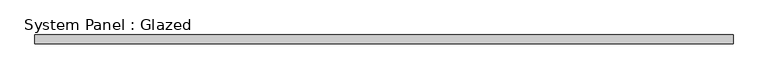
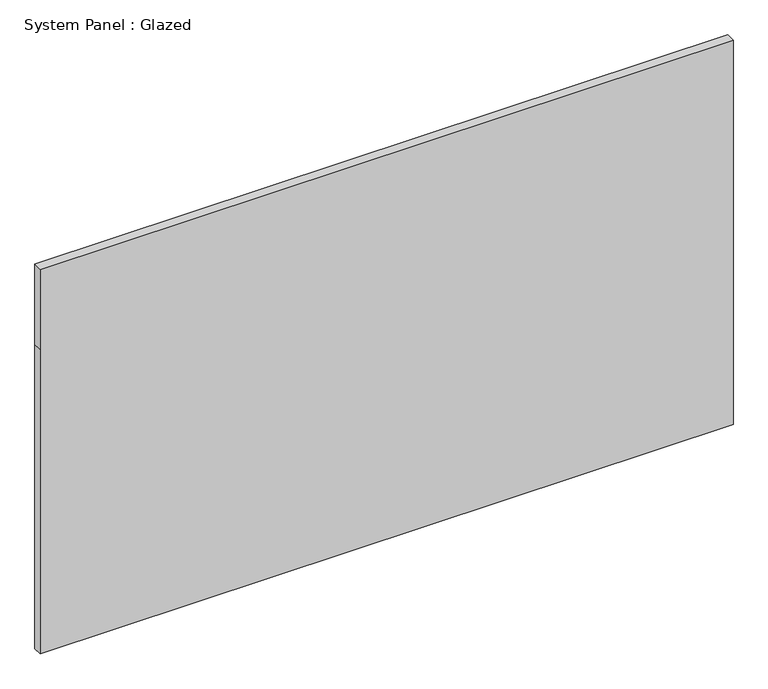
"""IFC4 building model written with IfcOpenShell, lengths in millimetres: plate geometry, System Panel : Glazed."""

from ifc_helpers import new_model, si_unit, frame, origin, place, context, project, spatial, polyline, outline, extrude, source, transform, mapped, element, save


def system_panel_glazed_3ba8046e(model_context):
    return source(origin(), model_context, "Body", "SweptSolid", [
        extrude(outline(polyline([(0.0, -984.25), (0.0, 984.25), (914.4, 984.25), (1155.7, 984.25), (1155.7, -984.25), (914.4, -984.25), (0.0, -984.25)])), frame((0.0, 19.05, 0.0), z_axis=(0.0, 1.0, 0.0), x_axis=(0.0, 0.0, 1.0)), (0.0, 0.0, 1.0), 25.4),
    ])


if __name__ == "__main__":
    model = new_model("IFC4")
    model_context = context("Model", 3, world=origin())
    ifc_project = project(units=[si_unit("LENGTHUNIT", "METRE", prefix="MILLI")], contexts=[model_context])
    site = spatial("IfcSite", under=ifc_project)
    building = spatial("IfcBuilding", under=site)
    placement = place(None, origin())
    system_panel_glazed_shape = system_panel_glazed_3ba8046e(model_context)
    element("IfcPlate", 1, ObjectType="System Panel : Glazed", at=placement, inside=building, context=model_context, shape_type="MappedRepresentation", body=[
        mapped(system_panel_glazed_shape, transform((0.0, 0.0, 0.0), x_axis=(1.0, 0.0, 0.0), y_axis=(0.0, 1.0, 0.0), z_axis=(0.0, 0.0, 1.0))),
    ])
    save(model, "model.ifc")

# Revit data of these elements
# Element 1 (IfcPlate, "System Panel : Glazed")
#   Materials on its faces: "Glass"
# Materials
#   "Glass": class "Glass", colour RGB 0 128 192, transparency 0.75
